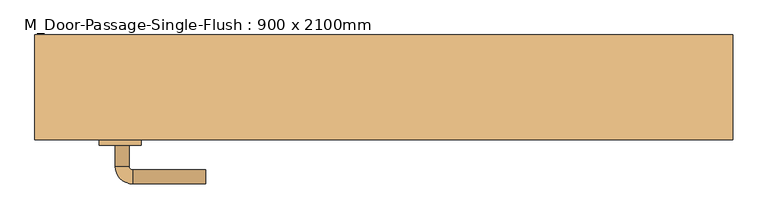
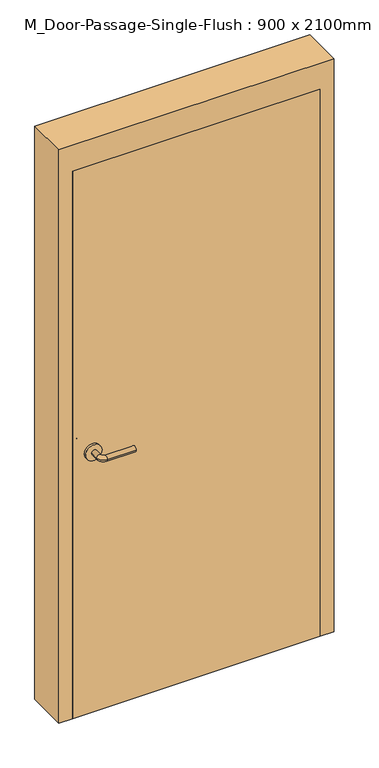
"""IFC4 building model written with IfcOpenShell, lengths in millimetres: door geometry, M_Door-Passage-Single-Flush : 900 x 2100mm."""

from ifc_helpers import new_model, si_unit, point, frame, frame_2d, origin, origin_with_axes, place, context, project, spatial, polyline, circle_curve, ellipse_curve, trimmed, segment, composite_curve, outline, extrude, faceted_brep, source, transform, mapped, element, save
from ifc_brep_helpers import plane_surface, cylinder_surface, revolved_surface, advanced_brep


def m_door_passage_single_flush_900_x_2100mm_89322b7b(model_context):
    return source(origin(), model_context, "Body", "SolidModel", [
        advanced_brep(
        [(-384.990625, -3.35, 1000.0), (-364.990625, -3.35, 1000.0), (-384.990625, 26.65, 1000.0), (-364.990625, 26.65, 1000.0), (-359.990625, 31.65, 1000.0), (-359.990625, 51.65, 1000.0), (-254.990625, 51.65, 1000.0), (-254.990625, 31.65, 1000.0)],
        [
            (0, 1, circle_curve(frame((-374.990625, -3.35, 1000.0), z_axis=(0.0, -1.0, 0.0), x_axis=(1.0, 0.0, 0.0)), 10.0)),
            (1, 0, circle_curve(frame((-374.990625, -3.35, 1000.0), z_axis=(0.0, -1.0, 0.0), x_axis=(1.0, 0.0, 0.0)), 10.0)),
            (0, 2),
            (2, 3, circle_curve(frame((-374.990625, 26.65, 1000.0), z_axis=(0.0, -1.0, 0.0), x_axis=(1.0, 0.0, 0.0)), 10.0)),
            (3, 1),
            (3, 2, circle_curve(frame((-374.990625, 26.65, 1000.0), z_axis=(0.0, -1.0, 0.0), x_axis=(1.0, 0.0, 0.0)), 10.0)),
            (4, 3, circle_curve(frame((-359.990625, 26.65, 1000.0), z_axis=(0.0, 0.0, 1.0), x_axis=(-1.0, 0.0, 0.0)), 5.0)),
            (2, 5, circle_curve(frame((-359.990625, 26.65, 1000.0), z_axis=(0.0, 0.0, -1.0), x_axis=(-1.0, 0.0, 0.0)), 25.0)),
            (5, 4, circle_curve(frame((-359.990625, 41.65, 1000.0), z_axis=(-1.0, 0.0, 0.0), x_axis=(0.0, -1.0, 0.0)), 10.0)),
            (4, 5, circle_curve(frame((-359.990625, 41.65, 1000.0), z_axis=(-1.0, 0.0, 0.0), x_axis=(0.0, -1.0, 0.0)), 10.0)),
            (6, 7, circle_curve(frame((-254.990625, 41.65, 1000.0), z_axis=(1.0, 0.0, 0.0), x_axis=(0.0, -1.0, 0.0)), 10.0)),
            (7, 6, circle_curve(frame((-254.990625, 41.65, 1000.0), z_axis=(1.0, 0.0, 0.0), x_axis=(0.0, -1.0, 0.0)), 10.0)),
            (5, 6),
            (7, 4),
        ],
        [
            plane_surface(frame((-374.990625, -3.35, 1000.0), z_axis=(0.0, -1.0, 0.0), x_axis=(0.0, 0.0, 1.0))),
            cylinder_surface(frame((-374.990625, -3.35, 1000.0), z_axis=(0.0, -1.0, 0.0), x_axis=(1.0, 0.0, 0.0)), 10.0),
            revolved_surface(trimmed(ellipse_curve(frame((-374.990625, 26.65, 1000.0), z_axis=(0.0, -1.0, 0.0), x_axis=(1.0, 0.0, 0.0)), 10.0, 10.0), [point((-384.990625, 26.65, 1000.0))], [point((-364.990625, 26.65, 1000.0))], True, "CARTESIAN"), (-359.990625, 26.65, 1000.0), (0.0, 0.0, -1.0)),
            revolved_surface(trimmed(ellipse_curve(frame((-374.990625, 26.65, 1000.0), z_axis=(0.0, -1.0, 0.0), x_axis=(1.0, 0.0, 0.0)), 10.0, 10.0), [point((-364.990625, 26.65, 1000.0))], [point((-384.990625, 26.65, 1000.0))], True, "CARTESIAN"), (-359.990625, 26.65, 1000.0), (0.0, 0.0, -1.0)),
            plane_surface(frame((-254.990625, 41.65, 1000.0), z_axis=(1.0, 0.0, 0.0), x_axis=(0.0, 0.0, 1.0))),
            cylinder_surface(frame((-359.990625, 41.65, 1000.0), z_axis=(-1.0, 0.0, 0.0), x_axis=(0.0, -1.0, 0.0)), 10.0),
        ],
        [
            (0, [[1, 2]]),
            (1, [[-1, 3, 4, 5]]),
            (1, [[-2, -5, 6, -3]]),
            (2, [[7, -4, 8, 9]]),
            (3, [[-8, -6, -7, 10]]),
            (4, [[11, 12]]),
            (5, [[-9, 13, -12, 14]]),
            (5, [[-10, -14, -11, -13]]),
        ],
    ),
        extrude(outline(composite_curve([segment(trimmed(circle_curve(frame_2d((1000.0, -377.490625)), 30.0), [point((1000.0, -407.490625))], [point((1000.0, -347.490625))], False, "CARTESIAN"), True, "CONTINUOUS"), segment(trimmed(circle_curve(frame_2d((1000.0, -377.490625)), 30.0), [point((1000.0, -347.490625))], [point((1000.0, -407.490625))], False, "CARTESIAN"), True, "CONTINUOUS")], self_intersect=False)), frame((0.0, -11.35, 0.0), z_axis=(0.0, 1.0, 0.0), x_axis=(0.0, 0.0, 1.0)), (0.0, 0.0, 1.0), 8.0),
        advanced_brep(
        [(-384.990625, -64.35, 1000.0), (-364.990625, -64.35, 1000.0), (-364.990625, -94.35, 1000.0), (-384.990625, -94.35, 1000.0), (-359.990625, -99.35, 1000.0), (-359.990625, -119.35, 1000.0), (-254.990625, -119.35, 1000.0), (-254.990625, -99.35, 1000.0)],
        [
            (0, 1, circle_curve(frame((-374.990625, -64.35, 1000.0), z_axis=(0.0, 1.0, 0.0), x_axis=(1.0, 0.0, 0.0)), 10.0)),
            (1, 0, circle_curve(frame((-374.990625, -64.35, 1000.0), z_axis=(0.0, 1.0, 0.0), x_axis=(1.0, 0.0, 0.0)), 10.0)),
            (1, 2),
            (2, 3, circle_curve(frame((-374.990625, -94.35, 1000.0), z_axis=(0.0, 1.0, 0.0), x_axis=(1.0, 0.0, 0.0)), 10.0)),
            (3, 0),
            (3, 2, circle_curve(frame((-374.990625, -94.35, 1000.0), z_axis=(0.0, 1.0, 0.0), x_axis=(1.0, 0.0, 0.0)), 10.0)),
            (4, 5, circle_curve(frame((-359.990625, -109.35, 1000.0), z_axis=(-1.0, 0.0, 0.0), x_axis=(0.0, 1.0, 0.0)), 10.0)),
            (5, 3, circle_curve(frame((-359.990625, -94.35, 1000.0), z_axis=(0.0, 0.0, -1.0), x_axis=(-1.0, 0.0, 0.0)), 25.0)),
            (2, 4, circle_curve(frame((-359.990625, -94.35, 1000.0), z_axis=(0.0, 0.0, 1.0), x_axis=(-1.0, 0.0, 0.0)), 5.0)),
            (5, 4, circle_curve(frame((-359.990625, -109.35, 1000.0), z_axis=(-1.0, 0.0, 0.0), x_axis=(0.0, 1.0, 0.0)), 10.0)),
            (6, 7, circle_curve(frame((-254.990625, -109.35, 1000.0), z_axis=(1.0, 0.0, 0.0), x_axis=(0.0, 1.0, 0.0)), 10.0)),
            (7, 6, circle_curve(frame((-254.990625, -109.35, 1000.0), z_axis=(1.0, 0.0, 0.0), x_axis=(0.0, 1.0, 0.0)), 10.0)),
            (4, 7),
            (6, 5),
        ],
        [
            plane_surface(frame((-374.990625, -64.35, 1000.0), z_axis=(0.0, 1.0, 0.0), x_axis=(0.0, 0.0, 1.0))),
            cylinder_surface(frame((-374.990625, -64.35, 1000.0), z_axis=(0.0, 1.0, 0.0), x_axis=(1.0, 0.0, 0.0)), 10.0),
            revolved_surface(trimmed(ellipse_curve(frame((-374.990625, -94.35, 1000.0), z_axis=(0.0, -1.0, 0.0), x_axis=(1.0, 0.0, 0.0)), 10.0, 10.0), [point((-384.990625, -94.35, 1000.0))], [point((-364.990625, -94.35, 1000.0))], True, "CARTESIAN"), (-359.990625, -94.35, 1000.0), (0.0, 0.0, -1.0)),
            revolved_surface(trimmed(ellipse_curve(frame((-374.990625, -94.35, 1000.0), z_axis=(0.0, -1.0, 0.0), x_axis=(1.0, 0.0, 0.0)), 10.0, 10.0), [point((-364.990625, -94.35, 1000.0))], [point((-384.990625, -94.35, 1000.0))], True, "CARTESIAN"), (-359.990625, -94.35, 1000.0), (0.0, 0.0, -1.0)),
            plane_surface(frame((-254.990625, -109.35, 1000.0), z_axis=(1.0, 0.0, 0.0), x_axis=(0.0, 0.0, 1.0))),
            cylinder_surface(frame((-359.990625, -109.35, 1000.0), z_axis=(-1.0, 0.0, 0.0), x_axis=(0.0, 1.0, 0.0)), 10.0),
        ],
        [
            (0, [[1, 2]]),
            (1, [[3, 4, 5, -2]]),
            (1, [[-5, 6, -3, -1]]),
            (2, [[7, 8, -4, 9]]),
            (3, [[10, -9, -6, -8]]),
            (4, [[11, 12]]),
            (5, [[13, -11, 14, -7]]),
            (5, [[-14, -12, -13, -10]]),
        ],
    ),
        extrude(outline(composite_curve([segment(trimmed(circle_curve(frame_2d((1000.0, -377.490625)), 30.0), [point((1000.0, -407.490625))], [point((1000.0, -347.490625))], False, "CARTESIAN"), True, "CONTINUOUS"), segment(trimmed(circle_curve(frame_2d((1000.0, -377.490625)), 30.0), [point((1000.0, -347.490625))], [point((1000.0, -407.490625))], False, "CARTESIAN"), True, "CONTINUOUS")], self_intersect=False)), frame((0.0, -64.35, 0.0), z_axis=(0.0, 1.0, 0.0), x_axis=(0.0, 0.0, 1.0)), (0.0, 0.0, 1.0), 8.0),
        extrude(outline(polyline([(450.0, -11.35), (450.0, -56.35), (-450.0, -56.35), (-450.0, -11.35), (450.0, -11.35)])), origin_with_axes(), (0.0, 0.0, 1.0), 2100.0),
        faceted_brep([(450.0, -6.5875, 0.0), (434.125, -6.5875, 0.0), (434.125, 44.4375, 0.0), (450.0, 44.4375, 0.0), (450.0, 93.65, 0.0), (500.0, 93.65, 0.0), (500.0, -56.35, 0.0), (450.0, -56.35, 0.0), (450.0, -56.35, 2100.0), (450.0, -6.5875, 2100.0), (500.0, -56.35, 2200.0), (-500.0, -56.35, 2200.0), (-500.0, -56.35, 0.0), (-450.0, -56.35, 0.0), (-450.0, -56.35, 2100.0), (500.0, 93.65, 2200.0), (450.0, 93.65, 2100.0), (-450.0, 93.65, 2100.0), (-450.0, 93.65, 0.0), (-500.0, 93.65, 0.0), (-500.0, 93.65, 2200.0), (450.0, 44.4375, 2100.0), (434.125, 44.4375, 2084.125), (-434.125, 44.4375, 2084.125), (-434.125, 44.4375, 0.0), (-450.0, 44.4375, 0.0), (-450.0, 44.4375, 2100.0), (434.125, -6.5875, 2084.125), (-450.0, -6.5875, 2100.0), (-450.0, -6.5875, 0.0), (-434.125, -6.5875, 0.0), (-434.125, -6.5875, 2084.125)], [[[0, 1, 2, 3, 4, 5, 6, 7]], [[7, 8, 9, 0]], [[6, 10, 11, 12, 13, 14, 8, 7]], [[5, 15, 10, 6]], [[4, 16, 17, 18, 19, 20, 15, 5]], [[3, 21, 16, 4]], [[2, 22, 23, 24, 25, 26, 21, 3]], [[1, 27, 22, 2]], [[0, 9, 28, 29, 30, 31, 27, 1]], [[8, 14, 28, 9]], [[16, 21, 26, 17]], [[22, 27, 31, 23]], [[12, 19, 18, 25, 24, 30, 29, 13]], [[13, 29, 28, 14]], [[11, 20, 19, 12]], [[17, 26, 25, 18]], [[23, 31, 30, 24]], [[15, 20, 11, 10]]]),
    ])


if __name__ == "__main__":
    model = new_model("IFC4")
    model_context = context("Model", 3, world=origin())
    ifc_project = project(units=[si_unit("LENGTHUNIT", "METRE", prefix="MILLI")], contexts=[model_context])
    site = spatial("IfcSite", under=ifc_project)
    building = spatial("IfcBuilding", under=site)
    placement = place(None, origin())
    m_door_passage_single_flush_900_x_2100mm_shape = m_door_passage_single_flush_900_x_2100mm_89322b7b(model_context)
    element("IfcDoor", 1, ObjectType="M_Door-Passage-Single-Flush : 900 x 2100mm", at=placement, inside=building, context=model_context, shape_type="MappedRepresentation", body=[
        mapped(m_door_passage_single_flush_900_x_2100mm_shape, transform((0.0, 0.0, 0.0), x_axis=(1.0, 0.0, 0.0), y_axis=(0.0, 1.0, 0.0), z_axis=(0.0, 0.0, 1.0))),
    ])
    save(model, "model.ifc")

# Revit data of these elements
# Type "M_Door-Passage-Single-Flush : 900 x 2100mm"
#   Type Mark = "38"
#   Analytic Construction = "Wooden"
#   Thickness = 45 mm
#   Thermal Resistance (R) = 0.455703 (m²·K)/W
#   Swing Angle [instance default] = 90.00°
#   Strike Height = 1000 mm
#   Rough Width [instance default] = 1000 mm
#   Rough Height [instance default] = 2200 mm
#   MF Opening Height [instance default] = 100 mm
#   MF Opening Width [instance default] = 100 mm
#   Inset Calculate [instance default] = 105 mm
#   Masonry Inset [instance default] = 25 mm
#   Height = 2100 mm
#   Width = 900 mm
#   Heat Transfer Coefficient (U) = 2.19465 W/(m²·K)
#   Masonry Frame Depth = 150 mm
#   Masonry Frame [instance default] = yes
#   Function = 1
#   Dry Wall Frame [instance default] = no
#   Panel Material = Wood - Birch
#   Frame Material = Metal - Paint Finish - Grey
#   Door Handle Material = Aluminum
#   Visual Light Transmittance = 0
#   Solar Heat Gain Coefficient = 0
#   Wall Closure = (empty or 0)
# Element 1 (IfcDoor, "M_Door-Passage-Single-Flush : 900 x 2100mm")
#   Materials on its faces: "Aluminum", "Metal - Paint Finish - Grey", "Wood - Birch"
# Materials
#   "Wood - Birch": class "Wood", colour RGB 173 132 96, transparency 0, Cost = 0
#   "Metal - Paint Finish - Grey": class "Paint", colour RGB 178 178 178, transparency 0, Cost = 0
#   "Aluminum": class "Metal", colour RGB 244 245 246, transparency 0, Description = "Aluminum 6061", Cost = 0
